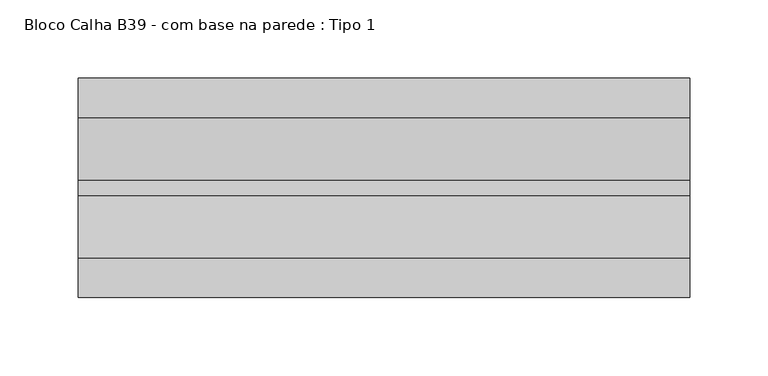
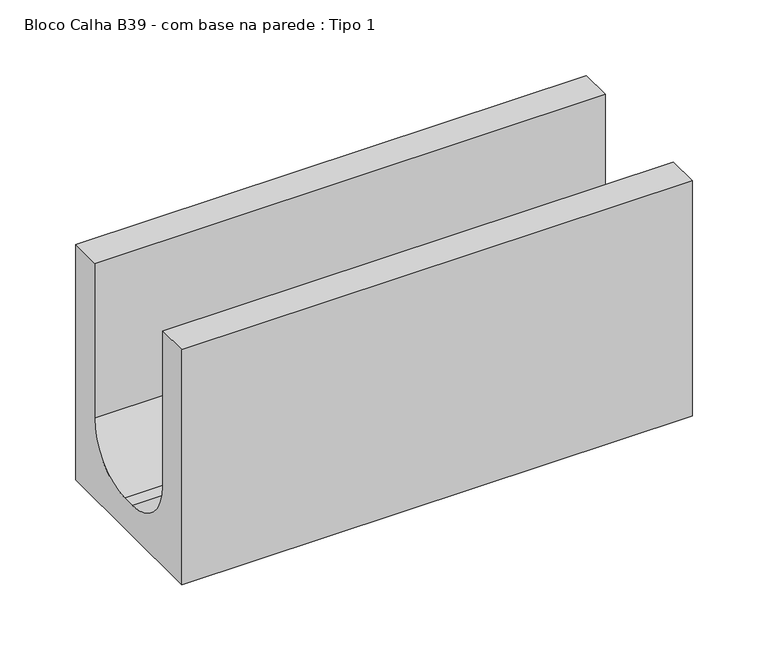
"""IFC4 building model written with IfcOpenShell, lengths in millimetres: proxy geometry, Bloco Calha B39 - com base na parede : Tipo 1."""

from ifc_helpers import new_model, si_unit, point, frame, frame_2d, origin, place, context, project, spatial, polyline, circle_curve, trimmed, segment, composite_curve, outline, extrude, source, transform, mapped, element, save


def bloco_calha_b39_com_base_na_parede_tipo_1_c44e9d18(model_context):
    return source(origin(), model_context, "Body", "SweptSolid", [
        extrude(outline(composite_curve([segment(polyline([(-70.0, 0.0), (-70.0, 190.0), (-45.0, 190.0), (-45.0, 65.0)]), True, "CONTINUOUS"), segment(trimmed(circle_curve(frame_2d((-5.0, 65.0)), 40.0), [point((-45.0, 65.0))], [point((-5.0, 25.0))], True, "CARTESIAN"), True, "CONTINUOUS"), segment(polyline([(-5.0, 25.0), (5.0, 25.0)]), True, "CONTINUOUS"), segment(trimmed(circle_curve(frame_2d((5.0, 65.0)), 40.0), [point((5.0, 25.0))], [point((45.0, 65.0))], True, "CARTESIAN"), True, "CONTINUOUS"), segment(polyline([(45.0, 65.0), (45.0, 190.0), (70.0, 190.0), (70.0, 0.0), (-70.0, 0.0)]), True, "CONTINUOUS")], self_intersect=False)), frame((-70.0, 0.0, 0.0), z_axis=(1.0, 0.0, 0.0), x_axis=(0.0, 1.0, 0.0)), (0.0, 0.0, 1.0), 390.0),
    ])


if __name__ == "__main__":
    model = new_model("IFC4")
    model_context = context("Model", 3, world=origin())
    ifc_project = project(units=[si_unit("LENGTHUNIT", "METRE", prefix="MILLI")], contexts=[model_context])
    site = spatial("IfcSite", under=ifc_project)
    building = spatial("IfcBuilding", under=site)
    placement = place(None, origin())
    bloco_calha_b39_com_base_na_parede_tipo_1_shape = bloco_calha_b39_com_base_na_parede_tipo_1_c44e9d18(model_context)
    element("IfcBuildingElementProxy", 1, Name="Bloco Calha B39 - com base na parede : Tipo 1", ObjectType="Bloco Calha B39 - com base na parede : Tipo 1", at=placement, inside=building, context=model_context, shape_type="MappedRepresentation", body=[
        mapped(bloco_calha_b39_com_base_na_parede_tipo_1_shape, transform((0.0, 0.0, 0.0), x_axis=(1.0, 0.0, 0.0), y_axis=(0.0, 1.0, 0.0), z_axis=(0.0, 0.0, 1.0))),
    ])
    save(model, "model.ifc")

# Revit data of these elements
# Type "Bloco Calha B39 - com base na parede : Tipo 1"
#   SINAPI = ""
#   Assembly Code = ""
